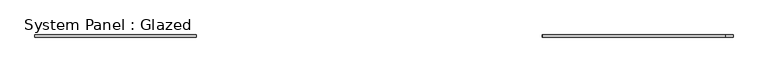
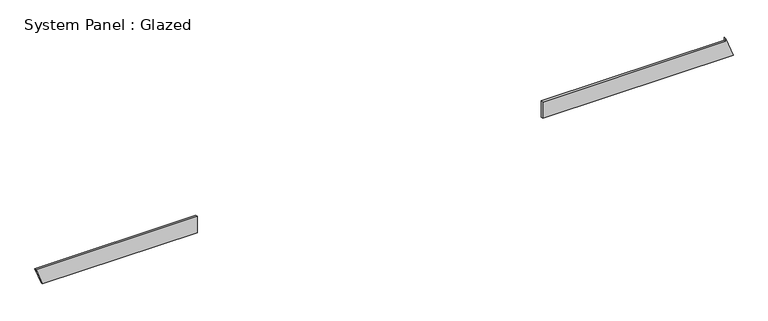
"""IFC4 building model written with IfcOpenShell, lengths in millimetres: plate geometry, System Panel : Glazed."""

from ifc_helpers import new_model, si_unit, frame, origin, place, context, project, spatial, polyline, outline, extrude, source, transform, mapped, element, save


def system_panel_glazed_948772bf(model_context):
    return source(origin(), model_context, "Body", "SweptSolid", [
        extrude(outline(polyline([(0.0, -3964.2777152), (0.0, -2170.9073948), (198.2936735, -2171.3320471), (198.4143393, -4035.2773263), (0.0, -3964.2777152)])), frame((0.0, -49.5, 0.0), z_axis=(0.0, 1.0, 0.0), x_axis=(0.0, 0.0, 1.0)), (0.0, 0.0, 1.0), 25.0),
        extrude(outline(polyline([(0.0, 1828.870126), (0.0, 4035.2773263), (233.2527248, 3950.1929605), (197.8973858, 3950.1906717), (198.0346921, 1829.1964261), (0.0, 1828.870126)])), frame((0.0, -49.5, 0.0), z_axis=(0.0, 1.0, 0.0), x_axis=(0.0, 0.0, 1.0)), (0.0, 0.0, 1.0), 25.0),
    ])


if __name__ == "__main__":
    model = new_model("IFC4")
    model_context = context("Model", 3, world=origin())
    ifc_project = project(units=[si_unit("LENGTHUNIT", "METRE", prefix="MILLI")], contexts=[model_context])
    site = spatial("IfcSite", under=ifc_project)
    building = spatial("IfcBuilding", under=site)
    placement = place(None, origin())
    system_panel_glazed_shape = system_panel_glazed_948772bf(model_context)
    element("IfcPlate", 1, ObjectType="System Panel : Glazed", at=placement, inside=building, context=model_context, shape_type="MappedRepresentation", body=[
        mapped(system_panel_glazed_shape, transform((0.0, 0.0, 0.0), x_axis=(1.0, 0.0, 0.0), y_axis=(0.0, 1.0, 0.0), z_axis=(0.0, 0.0, 1.0))),
    ])
    save(model, "model.ifc")

# Revit data of these elements
# Element 1 (IfcPlate, "System Panel : Glazed")
#   Materials on its faces: "Glass"
# Materials
#   "Glass": class "Glass", colour RGB 218 227 224, transparency 0.85, Description = "Soda Lime Glass", Cost = 0
